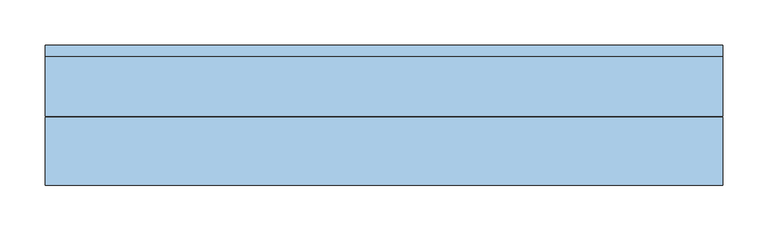
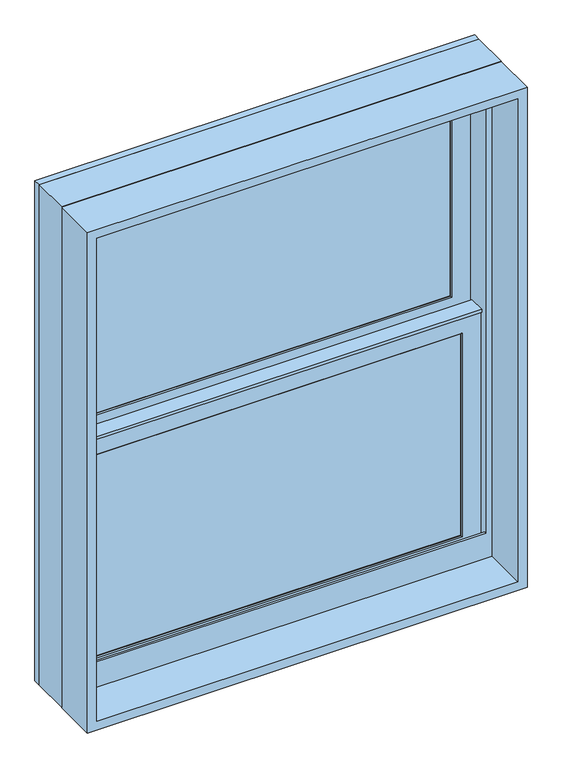
"""IFC4 building model written with IfcOpenShell, lengths in millimetres: window geometry, Window-Double_Hung-Marvin-Essential : ESDH2630."""

from ifc_helpers import new_model, si_unit, frame, origin, place, context, project, spatial, polyline, outline, extrude, faceted_brep, source, transform, mapped, element, save


def window_679e79a4(model_context):
    return source(origin(), model_context, "Body", "SolidModel", [
        extrude(outline(polyline([(115.3583333, 20.6375), (115.3583333, 15.875), (96.3083333, 15.875), (96.3083333, 20.6375), (115.3583333, 20.6375)])), frame((0.0, 0.0, 1593.85), z_axis=(0.0, 0.0, 1.0), x_axis=(1.0, 0.0, 0.0)), (0.0, 0.0, 1.0), 374.65),
        extrude(outline(polyline([(-96.3083333, 20.6375), (-96.3083333, 15.875), (-115.3583333, 15.875), (-115.3583333, 20.6375), (-96.3083333, 20.6375)])), frame((0.0, 0.0, 1593.85), z_axis=(0.0, 0.0, 1.0), x_axis=(1.0, 0.0, 0.0)), (0.0, 0.0, 1.0), 374.65),
        extrude(outline(polyline([(317.5, 20.6375), (317.5, 15.875), (-317.5, 15.875), (-317.5, 20.6375), (317.5, 20.6375)])), frame((0.0, 0.0, 1771.65), z_axis=(0.0, 0.0, 1.0), x_axis=(1.0, 0.0, 0.0)), (0.0, 0.0, 1.0), 19.05),
        extrude(outline(polyline([(-115.3583333, 46.83125), (-115.3583333, 51.59375), (-96.3083333, 51.59375), (-96.3083333, 46.83125), (-115.3583333, 46.83125)])), frame((0.0, 0.0, 2006.6), z_axis=(0.0, 0.0, 1.0), x_axis=(1.0, 0.0, 0.0)), (0.0, 0.0, 1.0), 374.65),
        extrude(outline(polyline([(96.3083333, 46.83125), (96.3083333, 51.59375), (115.3583333, 51.59375), (115.3583333, 46.83125), (96.3083333, 46.83125)])), frame((0.0, 0.0, 2006.6), z_axis=(0.0, 0.0, 1.0), x_axis=(1.0, 0.0, 0.0)), (0.0, 0.0, 1.0), 374.65),
        extrude(outline(polyline([(-317.5, 46.83125), (-317.5, 51.59375), (317.5, 51.59375), (317.5, 46.83125), (-317.5, 46.83125)])), frame((0.0, 0.0, 2184.4), z_axis=(0.0, 0.0, 1.0), x_axis=(1.0, 0.0, 0.0)), (0.0, 0.0, 1.0), 19.05),
        extrude(outline(polyline([(115.3583333, 20.6375), (96.3083333, 20.6375), (96.3083333, 25.4), (115.3583333, 25.4), (115.3583333, 20.6375)])), frame((0.0, 0.0, 1593.85), z_axis=(0.0, 0.0, 1.0), x_axis=(1.0, 0.0, 0.0)), (0.0, 0.0, 1.0), 374.65),
        extrude(outline(polyline([(-96.3083333, 20.6375), (-115.3583333, 20.6375), (-115.3583333, 25.4), (-96.3083333, 25.4), (-96.3083333, 20.6375)])), frame((0.0, 0.0, 1593.85), z_axis=(0.0, 0.0, 1.0), x_axis=(1.0, 0.0, 0.0)), (0.0, 0.0, 1.0), 374.65),
        extrude(outline(polyline([(317.5, 20.6375), (-317.5, 20.6375), (-317.5, 25.4), (317.5, 25.4), (317.5, 20.6375)])), frame((0.0, 0.0, 1771.65), z_axis=(0.0, 0.0, 1.0), x_axis=(1.0, 0.0, 0.0)), (0.0, 0.0, 1.0), 19.05),
        extrude(outline(polyline([(-115.3583333, 56.35625), (-96.3083333, 56.35625), (-96.3083333, 51.59375), (-115.3583333, 51.59375), (-115.3583333, 56.35625)])), frame((0.0, 0.0, 2006.6), z_axis=(0.0, 0.0, 1.0), x_axis=(1.0, 0.0, 0.0)), (0.0, 0.0, 1.0), 374.65),
        extrude(outline(polyline([(96.3083333, 56.35625), (115.3583333, 56.35625), (115.3583333, 51.59375), (96.3083333, 51.59375), (96.3083333, 56.35625)])), frame((0.0, 0.0, 2006.6), z_axis=(0.0, 0.0, 1.0), x_axis=(1.0, 0.0, 0.0)), (0.0, 0.0, 1.0), 374.65),
        extrude(outline(polyline([(-317.5, 56.35625), (317.5, 56.35625), (317.5, 51.59375), (-317.5, 51.59375), (-317.5, 56.35625)])), frame((0.0, 0.0, 2184.4), z_axis=(0.0, 0.0, 1.0), x_axis=(1.0, 0.0, 0.0)), (0.0, 0.0, 1.0), 19.05),
        faceted_brep([(-344.4875, 5.6780605, 1998.5351748), (-344.4875, 5.6780605, 1993.9), (344.4875, 5.6780605, 1993.9), (344.4875, 5.6780605, 1998.5351748), (-344.4875, 34.8118605, 1998.5351748), (344.4875, 34.8118605, 1998.5351748), (344.4875, 34.8118605, 1993.9), (-344.4875, 34.8118605, 1993.9), (-344.4875, 30.1625, 1993.9), (-344.4875, 30.1625, 1566.8625), (-344.4875, 8.9241104, 1566.8625), (-344.4875, 8.9241104, 1993.9), (344.4875, 8.9241104, 1993.9), (344.4875, 30.1625, 1993.9), (344.4875, 8.9241104, 1566.8625), (344.4875, 30.1625, 1566.8625), (-328.6034752, 11.90625, 1979.6034752), (-328.6034752, 30.1625, 1979.6034752), (328.6034752, 30.1625, 1979.6034752), (328.6034752, 11.90625, 1979.6034752), (-311.94375, 10.4662439, 1962.94375), (-311.94375, 11.90625, 1962.94375), (311.94375, 11.90625, 1962.94375), (311.94375, 10.4662439, 1962.94375), (313.4858834, 8.9241104, 1964.4858834), (-313.4858834, 8.9241104, 1964.4858834), (328.6034752, 30.1625, 1582.7465248), (328.6034752, 11.90625, 1582.7465248), (311.94375, 11.90625, 1599.40625), (311.94375, 10.4662439, 1599.40625), (313.4858834, 8.9241104, 1597.8641166), (-328.6034752, 30.1625, 1582.7465248), (-328.6034752, 11.90625, 1582.7465248), (-311.94375, 11.90625, 1599.40625), (-311.94375, 10.4662439, 1599.40625), (-313.4858834, 8.9241104, 1597.8641166)], [[[0, 1, 2, 3]], [[4, 5, 6, 7]], [[1, 0, 4, 7, 8, 9, 10, 11]], [[2, 1, 11, 12]], [[7, 6, 13, 8]], [[3, 2, 12, 14, 15, 13, 6, 5]], [[0, 3, 5, 4]], [[16, 17, 18, 19]], [[20, 21, 22, 23]], [[20, 23, 24, 25]], [[19, 18, 26, 27]], [[23, 22, 28, 29]], [[24, 23, 29, 30]], [[27, 26, 31, 32]], [[29, 28, 33, 34]], [[30, 29, 34, 35]], [[15, 14, 10, 9]], [[15, 9, 8, 13], [18, 17, 31, 26]], [[17, 16, 32, 31]], [[16, 19, 27, 32], [22, 21, 33, 28]], [[21, 20, 34, 33]], [[20, 25, 35, 34]], [[10, 14, 12, 11], [25, 24, 30, 35]]]),
        extrude(outline(polyline([(38.5955581, 1979.6125), (33.5778968, 1979.6125), (33.5778968, 1981.2), (39.9405976, 1981.2), (39.9405976, 1979.6125), (61.515625, 1979.6125), (47.6307501, 1976.2975159), (38.5955581, 1976.2975159), (38.5955581, 1979.6125)])), frame((-344.4875, 0.0, 0.0), z_axis=(1.0, 0.0, 0.0), x_axis=(0.0, 1.0, 0.0)), (0.0, 0.0, 1.0), 688.975),
        faceted_brep([(374.65, 0.0, 1536.7), (374.65, 0.0, 2438.4), (-374.65, 0.0, 2438.4), (-374.65, 0.0, 1536.7), (348.45625, 0.0, 1597.81875), (-348.45625, 0.0, 1597.81875), (-348.45625, 0.0, 2412.20625), (348.45625, 0.0, 2412.20625), (348.45625, 3.96875, 1536.7), (-348.45625, 3.96875, 1536.7), (-348.45625, 3.96875, 1597.81875), (348.45625, 3.96875, 1597.81875), (-374.65, 65.6828125, 1536.7), (-348.45625, 65.6828125, 1536.7), (348.45625, 65.6828125, 1536.7), (374.65, 65.6828125, 1536.7), (-374.65, 65.6828125, 2438.4), (374.65, 65.6828125, 2438.4), (348.45625, 65.6828125, 2412.20625), (-348.45625, 65.6828125, 2412.20625)], [[[0, 1, 2, 3], [4, 5, 6, 7]], [[8, 9, 10, 11]], [[5, 4, 11, 10]], [[0, 3, 12, 13, 9, 8, 14, 15]], [[13, 12, 16, 17, 15, 14, 18, 19]], [[13, 19, 6, 5, 10, 9]], [[7, 6, 19, 18]], [[18, 14, 8, 11, 4, 7]], [[1, 0, 15, 17]], [[2, 1, 17, 16]], [[3, 2, 16, 12]]]),
        faceted_brep([(348.45625, 30.1625, 1987.55), (346.86875, 30.1625, 1987.55), (346.86875, 30.1625, 1561.0544613), (348.45625, 30.1625, 1561.0544613), (-346.86875, 30.1625, 1987.55), (-348.45625, 30.1625, 1987.55), (-348.45625, 30.1625, 1561.0544613), (-346.86875, 30.1625, 1561.0544613), (346.86875, 63.5, 1987.55), (348.45625, 63.5, 1987.55), (348.45625, 63.5, 1554.5743077), (346.86875, 63.5, 1554.5743077), (-348.45625, 63.5, 1987.55), (-346.86875, 63.5, 1987.55), (-346.86875, 63.5, 1554.5743077), (-348.45625, 63.5, 1554.5743077), (359.7108932, 3.96875, 1566.1460105), (359.7108932, 3.96875, 1536.7), (359.7108932, 65.6828125, 1536.7), (359.7108932, 65.6828125, 1554.150012), (-359.7108932, 3.96875, 1536.7), (-359.7108932, 3.96875, 1566.1460105), (-359.7108932, 65.6828125, 1554.150012), (-359.7108932, 65.6828125, 1536.7), (359.7108932, 78.58125, 1551.6428097), (-359.7108932, 78.58125, 1551.6428097), (-357.6971252, 68.2348864, 1553.6539391), (-339.73135, 68.2348864, 1553.6539391), (-339.73135, 65.6828125, 1554.150012), (339.73135, 65.6828125, 1554.150012), (339.73135, 68.2348864, 1553.6539391), (357.6971252, 68.2348864, 1553.6539391), (-374.65, 65.6828125, 1536.7), (-374.65, 78.5948249, 1536.7), (374.65, 78.5948249, 1536.7), (374.65, 65.6828125, 1536.7), (-374.65, 78.58125, 2438.4), (374.65, 78.58125, 2438.4), (359.7108932, 78.58125, 2423.4608932), (-359.7108932, 78.58125, 2423.4608932), (-374.65, 65.6828125, 2438.4), (-357.6971252, 68.2348864, 2421.4471252), (357.6971252, 68.2348864, 2421.4471252), (339.73135, 68.2348864, 2403.48135), (-339.73135, 68.2348864, 2403.48135), (-339.73135, 65.6828125, 2403.48135), (339.73135, 65.6828125, 2403.48135), (374.65, 65.6828125, 2438.4)], [[[0, 1, 2, 3]], [[4, 5, 6, 7]], [[8, 9, 10, 11]], [[12, 13, 14, 15]], [[1, 8, 11, 2]], [[9, 0, 3, 10]], [[1, 0, 9, 8]], [[5, 4, 13, 12]], [[5, 12, 15, 6]], [[13, 4, 7, 14]], [[16, 17, 18, 19]], [[20, 21, 22, 23]], [[24, 25, 26, 27, 28, 22, 21, 16, 19, 29, 30, 31], [3, 2, 11, 10], [7, 6, 15, 14]], [[17, 16, 21, 20]], [[17, 20, 23, 32, 33, 34, 35, 18]], [[34, 33, 36, 37], [25, 24, 38, 39]], [[33, 32, 40, 36]], [[39, 41, 26, 25]], [[41, 42, 31, 30, 43, 44, 27, 26]], [[44, 45, 28, 27]], [[40, 32, 23, 22, 28, 45, 46, 29, 19, 18, 35, 47]], [[36, 40, 47, 37]], [[39, 38, 42, 41]], [[44, 43, 46, 45]], [[34, 37, 47, 35]], [[42, 38, 24, 31]], [[46, 43, 30, 29]]]),
        extrude(outline(polyline([(324.64375, 11.90625), (-324.64375, 11.90625), (-324.64375, 15.08125), (324.64375, 15.08125), (324.64375, 11.90625)])), frame((0.0, 0.0, 1586.70625), z_axis=(0.0, 0.0, 1.0), x_axis=(1.0, 0.0, 0.0)), (0.0, 0.0, 1.0), 388.9375),
        extrude(outline(polyline([(324.64375, 42.8625), (-324.64375, 42.8625), (-324.64375, 46.0375), (324.64375, 46.0375), (324.64375, 42.8625)])), frame((0.0, 0.0, 1999.45625), z_axis=(0.0, 0.0, 1.0), x_axis=(1.0, 0.0, 0.0)), (0.0, 0.0, 1.0), 388.9375),
        faceted_brep([(-311.94375, 31.194477, 1962.94375), (-313.4858834, 32.7366104, 1964.4858834), (313.4858834, 32.7366104, 1964.4858834), (311.94375, 31.194477, 1962.94375), (-311.94375, 30.1625, 1962.94375), (311.94375, 30.1625, 1962.94375), (-344.4875, 32.7366104, 1995.4875), (-344.4875, 30.1625, 1995.4875), (344.4875, 30.1625, 1995.4875), (344.4875, 32.7366104, 1995.4875), (313.4858834, 32.7366104, 1597.8641166), (311.94375, 31.194477, 1599.40625), (311.94375, 30.1625, 1599.40625), (344.4875, 30.1625, 1566.8625), (344.4875, 32.7366104, 1566.8625), (-313.4858834, 32.7366104, 1597.8641166), (-311.94375, 31.194477, 1599.40625), (-311.94375, 30.1625, 1599.40625), (-344.4875, 30.1625, 1566.8625), (-344.4875, 32.7366104, 1566.8625)], [[[0, 1, 2, 3]], [[4, 0, 3, 5]], [[6, 7, 8, 9]], [[3, 2, 10, 11]], [[5, 3, 11, 12]], [[9, 8, 13, 14]], [[11, 10, 15, 16]], [[12, 11, 16, 17]], [[14, 13, 18, 19]], [[9, 14, 19, 6], [1, 15, 10, 2]], [[16, 15, 1, 0]], [[17, 16, 0, 4]], [[7, 18, 13, 8], [5, 12, 17, 4]], [[19, 18, 7, 6]]]),
        faceted_brep([(-328.6034752, 42.8625, 2392.3534752), (-328.6034752, 61.11875, 2392.3534752), (328.6034752, 61.11875, 2392.3534752), (328.6034752, 42.8625, 2392.3534752), (-311.94375, 41.4224939, 2375.69375), (-311.94375, 42.8625, 2375.69375), (311.94375, 42.8625, 2375.69375), (311.94375, 41.4224939, 2375.69375), (-313.4858834, 39.8803604, 2377.2358834), (313.4858834, 39.8803604, 2377.2358834), (-344.4875, 61.11875, 2408.2375), (-344.4875, 39.8803604, 2408.2375), (344.4875, 39.8803604, 2408.2375), (344.4875, 61.11875, 2408.2375), (328.6034752, 61.11875, 1995.4965248), (328.6034752, 42.8625, 1995.4965248), (311.94375, 42.8625, 2012.15625), (311.94375, 41.4224939, 2012.15625), (313.4858834, 39.8803604, 2010.6141166), (344.4875, 39.8803604, 1979.6125), (344.4875, 61.11875, 1979.6125), (-328.6034752, 61.11875, 1995.4965248), (-328.6034752, 42.8625, 1995.4965248), (-311.94375, 42.8625, 2012.15625), (-311.94375, 41.4224939, 2012.15625), (-313.4858834, 39.8803604, 2010.6141166), (-344.4875, 39.8803604, 1979.6125), (-344.4875, 61.11875, 1979.6125)], [[[0, 1, 2, 3]], [[4, 5, 6, 7]], [[8, 4, 7, 9]], [[10, 11, 12, 13]], [[3, 2, 14, 15]], [[7, 6, 16, 17]], [[9, 7, 17, 18]], [[13, 12, 19, 20]], [[15, 14, 21, 22]], [[17, 16, 23, 24]], [[18, 17, 24, 25]], [[20, 19, 26, 27]], [[13, 20, 27, 10], [1, 21, 14, 2]], [[22, 21, 1, 0]], [[3, 15, 22, 0], [5, 23, 16, 6]], [[24, 23, 5, 4]], [[25, 24, 4, 8]], [[11, 26, 19, 12], [9, 18, 25, 8]], [[27, 26, 11, 10]]]),
        faceted_brep([(-344.4875, 61.11875, 1979.6125), (-344.4875, 63.6928604, 1979.6125), (344.4875, 63.6928604, 1979.6125), (344.4875, 61.11875, 1979.6125), (-311.94375, 62.150727, 2012.15625), (-311.94375, 61.11875, 2012.15625), (311.94375, 61.11875, 2012.15625), (311.94375, 62.150727, 2012.15625), (-313.4858834, 63.6928604, 2010.6141166), (313.4858834, 63.6928604, 2010.6141166), (344.4875, 63.6928604, 2408.2375), (344.4875, 61.11875, 2408.2375), (311.94375, 61.11875, 2375.69375), (311.94375, 62.150727, 2375.69375), (313.4858834, 63.6928604, 2377.2358834), (-344.4875, 63.6928604, 2408.2375), (-344.4875, 61.11875, 2408.2375), (-311.94375, 61.11875, 2375.69375), (-311.94375, 62.150727, 2375.69375), (-313.4858834, 63.6928604, 2377.2358834)], [[[0, 1, 2, 3]], [[4, 5, 6, 7]], [[8, 4, 7, 9]], [[3, 2, 10, 11]], [[7, 6, 12, 13]], [[9, 7, 13, 14]], [[11, 10, 15, 16]], [[13, 12, 17, 18]], [[14, 13, 18, 19]], [[16, 15, 1, 0]], [[3, 11, 16, 0], [5, 17, 12, 6]], [[18, 17, 5, 4]], [[19, 18, 4, 8]], [[1, 15, 10, 2], [9, 14, 19, 8]]]),
        extrude(outline(polyline([(324.64375, 26.19375), (-324.64375, 26.19375), (-324.64375, 30.1625), (324.64375, 30.1625), (324.64375, 26.19375)])), frame((0.0, 0.0, 1586.70625), z_axis=(0.0, 0.0, 1.0), x_axis=(1.0, 0.0, 0.0)), (0.0, 0.0, 1.0), 388.9375),
        extrude(outline(polyline([(324.64375, 57.15), (-324.64375, 57.15), (-324.64375, 61.11875), (324.64375, 61.11875), (324.64375, 57.15)])), frame((0.0, 0.0, 1999.45625), z_axis=(0.0, 0.0, 1.0), x_axis=(1.0, 0.0, 0.0)), (0.0, 0.0, 1.0), 388.9375),
        extrude(outline(polyline([(2438.4, 374.65), (2438.4, -374.65), (1536.7, -374.65), (1536.7, 374.65), (2438.4, 374.65)]), holes=[polyline([(2422.525, 358.775), (1552.575, 358.775), (1552.575, -358.775), (2422.525, -358.775), (2422.525, 358.775)])]), frame((0.0, -76.2, 0.0), z_axis=(0.0, 1.0, 0.0), x_axis=(0.0, 0.0, 1.0)), (0.0, 0.0, 1.0), 75.40625),
    ])


if __name__ == "__main__":
    model = new_model("IFC4")
    model_context = context("Model", 3, world=origin())
    ifc_project = project(units=[si_unit("LENGTHUNIT", "METRE", prefix="MILLI")], contexts=[model_context])
    site = spatial("IfcSite", under=ifc_project)
    building = spatial("IfcBuilding", under=site)
    placement = place(None, origin())
    window_shape = window_679e79a4(model_context)
    element("IfcWindow", 1, ObjectType="Window-Double_Hung-Marvin-Essential : ESDH2630", at=placement, inside=building, context=model_context, shape_type="MappedRepresentation", body=[
        mapped(window_shape, transform((0.0, 0.0, 0.0), x_axis=(1.0, 0.0, 0.0), y_axis=(0.0, 1.0, 0.0), z_axis=(0.0, 0.0, 1.0))),
    ])
    save(model, "model.ifc")

# Revit data of these elements
# Type "Window-Double_Hung-Marvin-Essential : ESDH2630"
#   Type Mark = "35"
#   Window Type = "Essential Double Hung"
#   Product data url = "https://bimobject.com/marvin-windows-and-doors/product/marvin-dhwau"
#   Product Guid = "c4a96547-874c-4385-91dc-a058adc19d98"
#   Frame = "All Ultrex"
#   Egress Window = "No"
#   URL = "www.marvin.com"
#   Model = "ESDH2630"
#   Manufacturer = "Marvin Windows and Doors"
#   Label Egress = ""
#   Glass Type = "IG Low E II with Argon"
#   Design Pressure = "DP50"
#   Description = "3036 DBHG"
#   Analytic Construction = "<None>"
#   Prairie Corner Width = 0' - 4"
#   Prairie Corner Height = 0' - 4"
#   Egress Width = 2' - 2 9/16"
#   Egress Height = 1' - 1 27/128"
#   Rough Width = 2' - 6"
#   Rough Height = 3' - 0"
#   Nominal Width = 2' - 6"
#   Nominal Height = 3' - 0"
#   Inset to Installation Flange [instance default] = 0' - 1"
#   Height = 2' - 11 1/2"
#   Egress Area = 2.43691 SF
#   Default Head Height = 8' - 0"
#   Width = 2' - 5 1/2"
#   Daylight Area = 4.88265 SF
#   DLO Width = 2' - 0 9/16"
#   DLO Height = 1' - 2 5/16"
#   Muntins Top Sash = yes
#   Lites Wide Top Sash = 3
#   Lites Wide Bottom Sash = 3
#   Lites High Top Sash = 2
#   Lites High Bottom Sash = 2
#   Lite Cut Prairie 9 = no
#   Lite Cut HV Grid = yes
#   Muntins Bottom Sash = yes
#   Label Visibility = no
#   Jamb Extension Visibility = yes
#   Edition number = 1
#   Interior Material = Ultrex-Marvin-Stonewhite
#   Glazing Material = Glass-Marvin-IG Low E II with Argon
#   Cladding Material = Ultrex-Marvin-Pebblegray
#   Wall Closure = (empty or 0)
#   Assembly Code = ""
# Element 1 (IfcWindow, "Window-Double_Hung-Marvin-Essential : ESDH2630")
#   Materials on its faces: "Ultrex-Marvin-Pebblegray", "Ultrex-Marvin-Stonewhite", "Glass-Marvin-IG Low E II with Argon"
# Materials
#   "Ultrex-Marvin-Stonewhite": class "Paint", colour RGB 250 251 245, transparency 0
#   "Glass-Marvin-IG Low E II with Argon": class "Glass", colour RGB 0 128 192, transparency 0.85
#   "Ultrex-Marvin-Pebblegray": class "Paint", colour RGB 189 185 173, transparency 0
